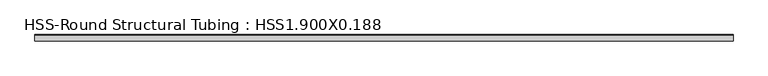
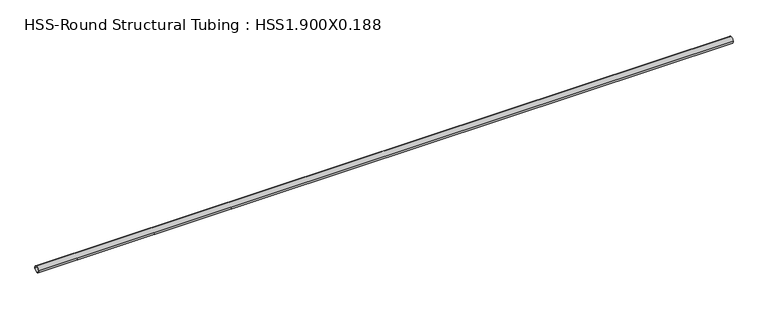
"""IFC4 building model written with IfcOpenShell, lengths in millimetres: member geometry, HSS-Round Structural Tubing : HSS1.900X0.188."""

from ifc_helpers import new_model, si_unit, point, frame, origin, origin_2d, place, context, project, spatial, circle_curve, trimmed, segment, composite_curve, outline, extrude, source, transform, mapped, element, save


def hss_round_structural_tubing_hss1_900x0_188_139ededb(model_context):
    return source(origin(), model_context, "Body", "SweptSolid", [
        extrude(outline(composite_curve([segment(trimmed(circle_curve(origin_2d(), 24.13), [point((-24.13, 0.0))], [point((24.13, 0.0))], False, "CARTESIAN"), True, "CONTINUOUS"), segment(trimmed(circle_curve(origin_2d(), 24.13), [point((24.13, 0.0))], [point((-24.13, 0.0))], False, "CARTESIAN"), True, "CONTINUOUS")], self_intersect=False), holes=[composite_curve([segment(trimmed(circle_curve(origin_2d(), 19.7104), [point((19.7104, 0.0))], [point((-19.7104, 0.0))], True, "CARTESIAN"), True, "CONTINUOUS"), segment(trimmed(circle_curve(origin_2d(), 19.7104), [point((-19.7104, 0.0))], [point((19.7104, 0.0))], True, "CARTESIAN"), True, "CONTINUOUS")], self_intersect=False)]), frame((-2747.8254285, 0.0, 0.0), z_axis=(1.0, 0.0, 0.0), x_axis=(0.0, 1.0, 0.0)), (0.0, 0.0, 1.0), 5329.4064562),
    ])


if __name__ == "__main__":
    model = new_model("IFC4")
    model_context = context("Model", 3, world=origin())
    ifc_project = project(units=[si_unit("LENGTHUNIT", "METRE", prefix="MILLI")], contexts=[model_context])
    site = spatial("IfcSite", under=ifc_project)
    building = spatial("IfcBuilding", under=site)
    placement = place(None, origin())
    hss_round_structural_tubing_hss1_900x0_188_shape = hss_round_structural_tubing_hss1_900x0_188_139ededb(model_context)
    element("IfcMember", 1, ObjectType="HSS-Round Structural Tubing : HSS1.900X0.188", at=placement, inside=building, context=model_context, shape_type="MappedRepresentation", body=[
        mapped(hss_round_structural_tubing_hss1_900x0_188_shape, transform((0.0, 0.0, 0.0), x_axis=(1.0, 0.0, 0.0), y_axis=(0.0, 1.0, 0.0), z_axis=(0.0, 0.0, 1.0))),
    ])
    save(model, "model.ifc")

# Revit data of these elements
# Type "HSS-Round Structural Tubing : HSS1.900X0.188"
#   Assembly Code = "B10"
#   t = 4.42 mm
#   W = 3.44
#   Length [instance default] = 1524 mm
#   OD = 48.26 mm
#   A = 0.000608386 m²
#   Structural Material [instance default] = Steel ASTM A500, Grade B, Round
# Element 1 (IfcMember, "HSS-Round Structural Tubing : HSS1.900X0.188")
#   Materials on its faces: "Steel ASTM A500, Grade B, Round"
# Materials
#   "Steel ASTM A500, Grade B, Round": class "Metal", colour RGB 199 199 199, transparency 0, Description = "Carbon steel", Cost = 0
